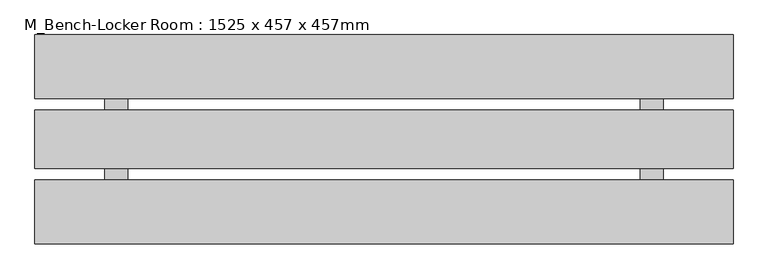
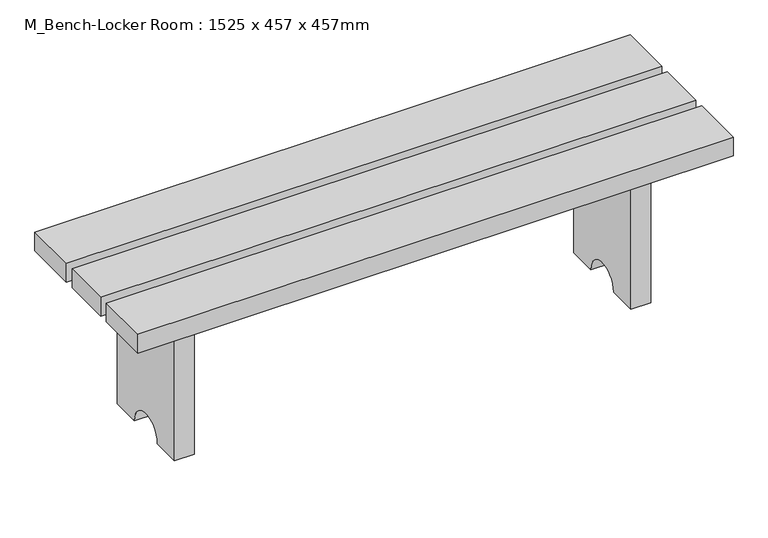
"""IFC4 building model written with IfcOpenShell, lengths in millimetres: furniture geometry, M_Bench-Locker Room : 1525 x 457 x 457mm."""

from ifc_helpers import new_model, si_unit, point, frame, frame_2d, origin, place, context, project, spatial, polyline, circle_curve, trimmed, segment, composite_curve, outline, extrude, source, transform, mapped, element, save


def m_bench_locker_room_1525_x_457_x_457mm_16fc9c3f(model_context):
    return source(origin(), model_context, "Body", "SweptSolid", [
        extrude(outline(composite_curve([segment(polyline([(-307.6147541, 0.0), (-307.6147541, 406.2), (-53.8147541, 406.2), (-53.8147541, 0.0), (-130.0147541, 0.0)]), True, "CONTINUOUS"), segment(trimmed(circle_curve(frame_2d((-180.7147541, 0.0)), 50.7), [point((-130.0147541, 0.0))], [point((-231.4147541, 0.0))], True, "CARTESIAN"), True, "CONTINUOUS"), segment(polyline([(-231.4147541, 0.0), (-307.6147541, 0.0)]), True, "CONTINUOUS")], self_intersect=False)), frame((403.9852459, 0.0, 0.0), z_axis=(1.0, 0.0, 0.0), x_axis=(0.0, 1.0, 0.0)), (0.0, 0.0, 1.0), 50.8),
        extrude(outline(composite_curve([segment(polyline([(-53.8147541, 0.0), (-130.0147541, 0.0)]), True, "CONTINUOUS"), segment(trimmed(circle_curve(frame_2d((-180.7147541, 0.0)), 50.7), [point((-130.0147541, 0.0))], [point((-231.4147541, 0.0))], True, "CARTESIAN"), True, "CONTINUOUS"), segment(polyline([(-231.4147541, 0.0), (-307.6147541, 0.0), (-307.6147541, 406.2), (-53.8147541, 406.2), (-53.8147541, 0.0)]), True, "CONTINUOUS")], self_intersect=False)), frame((-765.4147541, 0.0, 0.0), z_axis=(1.0, 0.0, 0.0), x_axis=(0.0, 1.0, 0.0)), (0.0, 0.0, 1.0), 50.8),
        extrude(outline(polyline([(607.1852459, 47.7852459), (607.1852459, -91.8480874), (-917.8147541, -91.8480874), (-917.8147541, 47.7852459), (607.1852459, 47.7852459)])), frame((0.0, 0.0, 406.2), z_axis=(0.0, 0.0, 1.0), x_axis=(1.0, 0.0, 0.0)), (0.0, 0.0, 1.0), 50.8),
        extrude(outline(polyline([(607.1852459, -409.2147541), (-917.8147541, -409.2147541), (-917.8147541, -269.5814208), (607.1852459, -269.5814208), (607.1852459, -409.2147541)])), frame((0.0, 0.0, 406.2), z_axis=(0.0, 0.0, 1.0), x_axis=(1.0, 0.0, 0.0)), (0.0, 0.0, 1.0), 50.8),
        extrude(outline(polyline([(607.1852459, -117.2480874), (607.1852459, -244.1814208), (-917.8147541, -244.1814208), (-917.8147541, -117.2480874), (607.1852459, -117.2480874)])), frame((0.0, 0.0, 406.2), z_axis=(0.0, 0.0, 1.0), x_axis=(1.0, 0.0, 0.0)), (0.0, 0.0, 1.0), 50.8),
    ])


if __name__ == "__main__":
    model = new_model("IFC4")
    model_context = context("Model", 3, world=origin())
    ifc_project = project(units=[si_unit("LENGTHUNIT", "METRE", prefix="MILLI")], contexts=[model_context])
    site = spatial("IfcSite", under=ifc_project)
    building = spatial("IfcBuilding", under=site)
    placement = place(None, origin())
    m_bench_locker_room_1525_x_457_x_457mm_shape = m_bench_locker_room_1525_x_457_x_457mm_16fc9c3f(model_context)
    element("IfcFurniture", 1, ObjectType="M_Bench-Locker Room : 1525 x 457 x 457mm", at=placement, inside=building, context=model_context, shape_type="MappedRepresentation", body=[
        mapped(m_bench_locker_room_1525_x_457_x_457mm_shape, transform((0.0, 0.0, 0.0), x_axis=(1.0, 0.0, 0.0), y_axis=(0.0, 1.0, 0.0), z_axis=(0.0, 0.0, 1.0))),
    ])
    save(model, "model.ifc")

# Revit data of these elements
# Type "M_Bench-Locker Room : 1525 x 457 x 457mm"
#   Depth = 0.457 m
#   Height = 0.457 m
#   Width = 1.525 m
#   Bench Material = Cherry
#   Default Elevation = 0
# Element 1 (IfcFurniture, "M_Bench-Locker Room : 1525 x 457 x 457mm")
#   Materials on its faces: "Cherry"
# Materials
#   "Cherry": class "Wood", colour RGB 157 77 38, transparency 0, Description = "Prunus Serotina", Cost = 0
